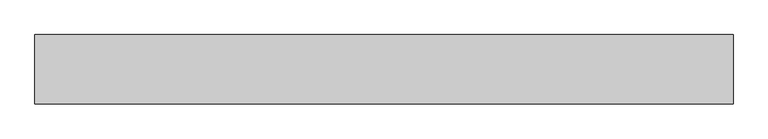
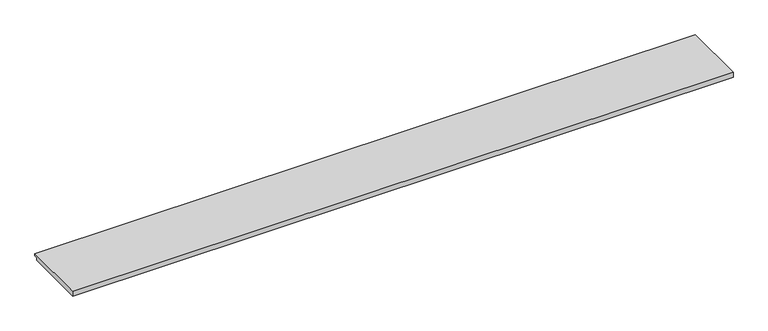
"""IFC4 building model written with IfcOpenShell, lengths in millimetres: proxy geometry, Generic Models 7:Generic Models 1:6:Generic Models 1:6 : Generic Models 7:Generic Models 1:337419:7 : Generic Models 7:Generic Models 1:6:Generic Models 1:6 : Generic Models 7:Generic Models 1:337419:312901."""

from ifc_helpers import new_model, si_unit, frame, origin, place, context, project, spatial, polyline, outline, extrude, source, transform, mapped, element, save


def generic_models_fe21daaa(model_context):
    return source(origin(), model_context, "Body", "SweptSolid", [
        extrude(outline(polyline([(-537134.457511, 0.0), (-537134.457511, 38.1), (-536651.2132902, 38.1), (-536651.2132902, 20.9771437), (-536675.8645285, 19.2533612), (-536675.8645285, 0.0), (-537134.457511, 0.0)])), frame((591306.0367242, 0.0, 0.0), z_axis=(1.0, 0.0, 0.0), x_axis=(0.0, 1.0, 0.0)), (0.0, 0.0, 1.0), 4876.8),
    ])


if __name__ == "__main__":
    model = new_model("IFC4")
    model_context = context("Model", 3, world=origin())
    ifc_project = project(units=[si_unit("LENGTHUNIT", "METRE", prefix="MILLI")], contexts=[model_context])
    site = spatial("IfcSite", under=ifc_project)
    building = spatial("IfcBuilding", under=site)
    placement = place(None, origin())
    generic_models_shape = generic_models_fe21daaa(model_context)
    element("IfcBuildingElementProxy", 1, Name="Generic Models 7:Generic Models 1:6:Generic Models 1:6 : Generic Models 7:Generic Models 1:337419:7 : Generic Models 7:Generic Models 1:6:Generic Models 1:6 : Generic Models 7:Generic Models 1:337419:312901", ObjectType="Generic Models 7:Generic Models 1:6:Generic Models 1:6 : Generic Models 7:Generic Models 1:337419:7 : Generic Models 7:Generic Models 1:6:Generic Models 1:6 : Generic Models 7:Generic Models 1:337419:312901", at=placement, inside=building, context=model_context, shape_type="MappedRepresentation", body=[
        mapped(generic_models_shape, transform((0.0, 0.0, 0.0), x_axis=(1.0, 0.0, 0.0), y_axis=(0.0, 1.0, 0.0), z_axis=(0.0, 0.0, 1.0))),
    ])
    save(model, "model.ifc")

# Revit data of these elements
# Type "Generic Models 7:Generic Models 1:6:Generic Models 1:6 : Generic Models 7:Generic Models 1:337419:7 : Generic Models 7:Generic Models 1:6:Generic Models 1:6 : Generic Models 7:Generic Models 1:337419:312901"
#   NameOverride = "Generic Models 7:Generic Models 1:6:Generic Models 1:6 : Generic Models 7:Generic Models 1:337419:312901"
#   ObjectTypeOverride = "Generic Models 1:6 : Generic Models 7:Generic Models 1:337419"
#   Reference = "Generic Models 1"
#   Tag = "312901"
# Element 1 (IfcBuildingElementProxy, "Generic Models 7:Generic Models 1:6:Generic Models 1:6 : Generic Models 7:Generic Models 1:337419:7 : Generic Models 7:Generic Models 1:6:Generic Models 1:6 : Generic Models 7:Generic Models 1:337419:312901")
#   Materials on its faces: "FLOOR FINISH - SEE FINISH PLAN"
# Materials
#   "FLOOR FINISH - SEE FINISH PLAN": class "Generic", colour RGB 220 194 213, transparency 0, Cost = 0
